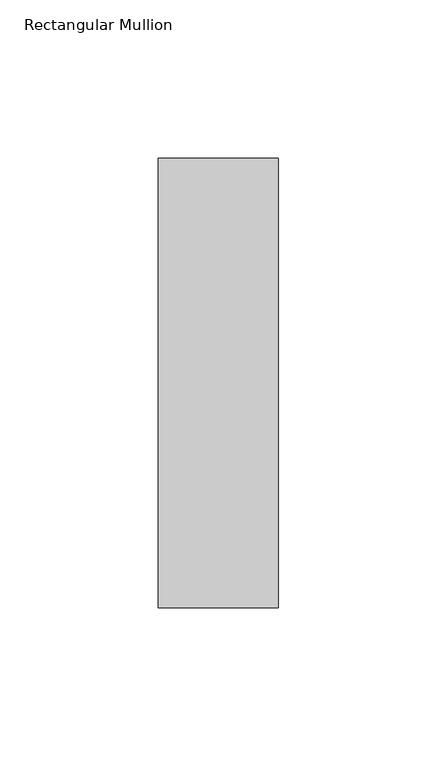
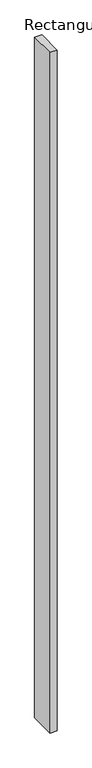
"""IFC4 building model written with IfcOpenShell, lengths in millimetres: member geometry, Rectangular Mullion : NLRS_21_CWM_hsb-regel 38x142_gen_rsf."""

from ifc_helpers import new_model, si_unit, frame, origin, place, context, project, spatial, polyline, outline, extrude, source, transform, mapped, element, save


def rectangular_mullion_d78042b4(model_context):
    return source(origin(), model_context, "Body", "SweptSolid", [
        extrude(outline(polyline([(-38.0, -71.0), (-38.0, 71.0), (0.0, 71.0), (0.0, -71.0), (-38.0, -71.0)])), frame((0.0, 0.0, -3849.0), z_axis=(0.0, 0.0, 1.0), x_axis=(1.0, 0.0, 0.0)), (0.0, 0.0, 1.0), 3849.0),
    ])


if __name__ == "__main__":
    model = new_model("IFC4")
    model_context = context("Model", 3, world=origin())
    ifc_project = project(units=[si_unit("LENGTHUNIT", "METRE", prefix="MILLI")], contexts=[model_context])
    site = spatial("IfcSite", under=ifc_project)
    building = spatial("IfcBuilding", under=site)
    placement = place(None, origin())
    rectangular_mullion_shape = rectangular_mullion_d78042b4(model_context)
    element("IfcMember", 1, ObjectType="Rectangular Mullion : NLRS_21_CWM_hsb-regel 38x142_gen_rsf", at=placement, inside=building, context=model_context, shape_type="MappedRepresentation", body=[
        mapped(rectangular_mullion_shape, transform((0.0, 0.0, 0.0), x_axis=(1.0, 0.0, 0.0), y_axis=(0.0, 1.0, 0.0), z_axis=(0.0, 0.0, 1.0))),
    ])
    save(model, "model.ifc")

# Revit data of these elements
# Type "Rectangular Mullion : NLRS_21_CWM_hsb-regel 38x142_gen_rsf"
#   Export Type to IFC As = "IfcWall"
#   Type IfcGUID = "07M7mRoiH1CR8m_RSKIwpF"
#   Assembly Code = "21.10"
#   built-in parameter 1007322 = 0.465879 (stored number, unit not read)
#   built-in parameter 1007321 = 0.062336 (stored number, unit not read)
#   built-in parameter 1007320 = 0.062336 (stored number, unit not read)
# Element 1 (IfcMember, "Rectangular Mullion : NLRS_21_CWM_hsb-regel 38x142_gen_rsf")
#   Materials on its faces: "NLRS_i2_hout naaldhout vuren_gen_rsf"
# Materials
#   "NLRS_i2_hout naaldhout vuren_gen_rsf": class "I - Hout", colour RGB 234 199 147, transparency 0, Keynote = "i2", Manufacturer = "Revit Standards Foundation", URL = "www.revitstandards.org", Description = "hout vuren", Cost = 0
